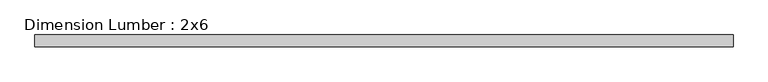
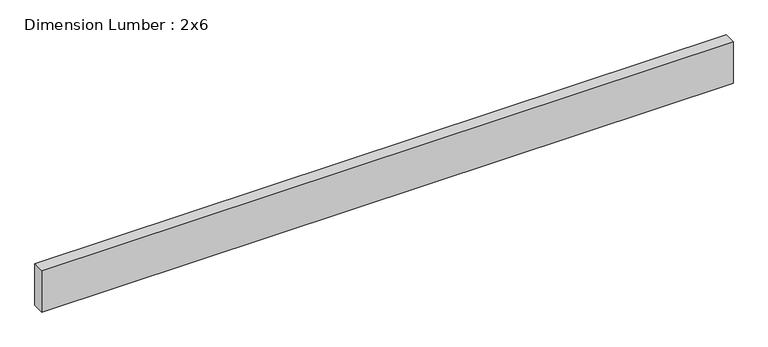
"""IFC4 building model written with IfcOpenShell, lengths in millimetres: beam geometry, Dimension Lumber : 2x6."""

import ifcopenshell
import ifcopenshell.guid

model = None  # the IFC model being written
_history = None  # IfcOwnerHistory: only IFC2X3 demands one
_inside = {}  # id of a spatial element -> (the spatial element, [elements in it])
_under = {}  # id of a project, library or spatial element -> (it, [spatial elements below it])
_declared = {}  # id of a project -> (the project, [libraries it declares])
_typed = {}  # id of a type object -> (the type object, [elements of that type])
_made_of = {}  # id of a material, layer set ... -> (it, [elements and type objects made of it])


def new_model(schema):
    """Start an empty IFC model of exactly this schema.

    Asked for "IFC4X3", IfcOpenShell would pick the latest addendum, in which some entities
    have other attributes; the version numbers below select the first issue.
    IFC2X3 requires an IfcOwnerHistory on every rooted entity: one is made here for all.
    """
    global model, _history
    if schema == "IFC4X3":
        model = ifcopenshell.file(schema_version=(4, 3, 0, 0))
    else:
        model = ifcopenshell.file(schema=schema)
    _inside.clear()
    _under.clear()
    _declared.clear()
    _typed.clear()
    _made_of.clear()
    _history = None
    if model.schema == "IFC2X3":
        org = make("IfcOrganization", Name="unknown")
        user = make(
            "IfcPersonAndOrganization",
            ThePerson=make("IfcPerson", FamilyName="unknown"),
            TheOrganization=org,
        )
        app = make(
            "IfcApplication",
            ApplicationDeveloper=org,
            Version="unknown",
            ApplicationFullName="unknown",
            ApplicationIdentifier="unknown",
        )
        _history = make(
            "IfcOwnerHistory",
            OwningUser=user,
            OwningApplication=app,
            ChangeAction="ADDED",
            CreationDate=0,
        )
    return model


def make(cls, **values):
    """One entity of the class cls with the attributes given. An attribute that is None is left unset."""
    return model.create_entity(
        cls, **{name: value for name, value in values.items() if value is not None}
    )


def rooted(cls, **values):
    """An entity with a GlobalId (a new one), such as an element, a storey or a relation."""
    return make(cls, GlobalId=ifcopenshell.guid.new(), OwnerHistory=_history, **values)


def si_unit(unit_type, name, prefix=None):
    """IfcSIUnit, for example si_unit("LENGTHUNIT", "METRE", prefix="MILLI")."""
    return make("IfcSIUnit", UnitType=unit_type, Prefix=prefix, Name=name)


def assignment(units):
    """IfcUnitAssignment: the units of a project."""
    return None if units is None else make("IfcUnitAssignment", Units=units)


def point(xyz):
    """IfcCartesianPoint."""
    return None if xyz is None else make("IfcCartesianPoint", Coordinates=xyz)


def direction(xyz):
    """IfcDirection."""
    return None if xyz is None else make("IfcDirection", DirectionRatios=xyz)


def frame(location, z_axis=None, x_axis=None):
    """IfcAxis2Placement3D, a coordinate frame: its origin and axes. An axis left out is left unset."""
    return make(
        "IfcAxis2Placement3D",
        Location=point(location),
        Axis=direction(z_axis),
        RefDirection=direction(x_axis),
    )


def origin():
    """The frame at (0, 0, 0) with its axes left unset."""
    return frame((0.0, 0.0, 0.0))


def place(relative_to, where):
    """IfcLocalPlacement: puts the frame where relative to a parent placement (None: the world)."""
    return make(
        "IfcLocalPlacement", PlacementRelTo=relative_to, RelativePlacement=where
    )


def context(
    kind, dimensions, precision=None, world=None, true_north=None, identifier=None
):
    """IfcGeometricRepresentationContext, for example the 3D "Model" context."""
    return make(
        "IfcGeometricRepresentationContext",
        ContextIdentifier=identifier,
        ContextType=kind,
        CoordinateSpaceDimension=dimensions,
        Precision=precision,
        WorldCoordinateSystem=world,
        TrueNorth=true_north,
    )


def project(units=None, contexts=None):
    """IfcProject with its units and contexts."""
    return rooted(
        "IfcProject",
        Name="project",
        RepresentationContexts=contexts,
        UnitsInContext=assignment(units),
    )


def spatial(cls, under=None, at=None, **own):
    """A site, building, storey or space (cls), placed at a placement, below another one or the project."""
    s = rooted(cls, ObjectPlacement=at, **own)
    if under is not None:
        _under.setdefault(under.id(), (under, []))[1].append(s)
    return s


def polyline(points):
    """IfcPolyline through the points."""
    return make("IfcPolyline", Points=[point(p) for p in points])


def outline(outer, holes=None, kind="AREA"):
    """IfcArbitraryClosedProfileDef: a profile drawn as a closed curve; with holes, ...WithVoids."""
    if holes is None:
        return make("IfcArbitraryClosedProfileDef", ProfileType=kind, OuterCurve=outer)
    return make(
        "IfcArbitraryProfileDefWithVoids",
        ProfileType=kind,
        OuterCurve=outer,
        InnerCurves=holes,
    )


def extrude(swept, where, along, depth):
    """IfcExtrudedAreaSolid: the profile swept, set in the frame where, extruded along a direction by depth."""
    return make(
        "IfcExtrudedAreaSolid",
        SweptArea=swept,
        Position=where,
        ExtrudedDirection=direction(along),
        Depth=depth,
    )


def shape(context_of_items, identifier, shape_type, items):
    """IfcShapeRepresentation: the items that make up one representation, for example the "Body"."""
    return make(
        "IfcShapeRepresentation",
        ContextOfItems=context_of_items,
        RepresentationIdentifier=identifier,
        RepresentationType=shape_type,
        Items=items,
    )


def source(mapping_origin, context_of_items, identifier, shape_type, items):
    """IfcRepresentationMap: a shape defined once, which mapped items show again and again."""
    return make(
        "IfcRepresentationMap",
        MappingOrigin=mapping_origin,
        MappedRepresentation=shape(context_of_items, identifier, shape_type, items),
    )


def transform(
    local_origin,
    x_axis=None,
    y_axis=None,
    z_axis=None,
    scale=None,
    scale2=None,
    scale3=None,
    uniform=True,
):
    """IfcCartesianTransformationOperator3D, or its non-uniform kind. x_axis, y_axis, z_axis: its Axis1, 2, 3."""
    if uniform:
        return make(
            "IfcCartesianTransformationOperator3D",
            Axis1=direction(x_axis),
            Axis2=direction(y_axis),
            LocalOrigin=point(local_origin),
            Scale=scale,
            Axis3=direction(z_axis),
        )
    return make(
        "IfcCartesianTransformationOperator3DnonUniform",
        Axis1=direction(x_axis),
        Axis2=direction(y_axis),
        LocalOrigin=point(local_origin),
        Scale=scale,
        Axis3=direction(z_axis),
        Scale2=scale2,
        Scale3=scale3,
    )


def mapped(mapping_source, mapping_target):
    """IfcMappedItem: shows the shape of a source again, moved by a transform."""
    return make(
        "IfcMappedItem", MappingSource=mapping_source, MappingTarget=mapping_target
    )


def made_of(thing, what):
    """Note that an element or type object is made of a material, layer set ...; save() writes the relation."""
    if what is not None:
        _made_of.setdefault(what.id(), (what, []))[1].append(thing)
    return thing


def element(
    cls,
    number,
    at=None,
    inside=None,
    cuts=None,
    type_object=None,
    material=None,
    context=None,
    identifier="Body",
    shape_type=None,
    held_by="IfcProductDefinitionShape",
    body=None,
    shapes=None,
    **own,
):
    """One element of the class cls, such as IfcWall. Its Tag is "e" and its number.

    at: its placement. inside: the storey or other place that contains it. cuts: it is an
    opening in that element (IfcRelVoidsElement). A single representation is given by context,
    identifier, shape_type and body (its items); several are given by shapes. held_by: the class
    of the entity that holds the representations. save() writes the other relations.
    """
    e = rooted(cls, Tag="e%d" % number, ObjectPlacement=at, **own)
    if body is not None:
        shapes = [shape(context, identifier, shape_type, body)]
    if shapes is not None:
        e.Representation = make(held_by, Representations=shapes)
    if inside is not None:
        _inside.setdefault(inside.id(), (inside, []))[1].append(e)
    if cuts is not None:
        rooted(
            "IfcRelVoidsElement", RelatingBuildingElement=cuts, RelatedOpeningElement=e
        )
    if type_object is not None:
        _typed.setdefault(type_object.id(), (type_object, []))[1].append(e)
    return made_of(e, material)


def aggregate(whole, parts):
    """IfcRelAggregates: a whole, such as a stair, and the parts it consists of."""
    return rooted("IfcRelAggregates", RelatingObject=whole, RelatedObjects=parts)


def save(model, path):
    """Write the relations noted so far, then the file.

    IfcRelAggregates (storeys below a building ...), IfcRelContainedInSpatialStructure (elements
    in a storey), IfcRelDefinesByType, IfcRelAssociatesMaterial and IfcRelDeclares: one each for
    every whole, place, type object, material and project.
    """
    for whole, parts in _under.values():
        aggregate(whole, parts)
    for where, things in _inside.values():
        rooted(
            "IfcRelContainedInSpatialStructure",
            RelatedElements=things,
            RelatingStructure=where,
        )
    for kind, things in _typed.values():
        rooted("IfcRelDefinesByType", RelatedObjects=things, RelatingType=kind)
    for what, things in _made_of.values():
        rooted("IfcRelAssociatesMaterial", RelatedObjects=things, RelatingMaterial=what)
    for by, libraries in _declared.values():
        rooted("IfcRelDeclares", RelatingContext=by, RelatedDefinitions=libraries)
    model.write(path)


def dimension_lumber_2x6_f4b49fb7(model_context):
    return source(origin(), model_context, "Body", "SweptSolid", [
        extrude(outline(polyline([(1700.453938, 19.05), (1700.453938, -19.05), (-505.9373564, -19.05), (-505.9373564, 19.05), (1700.453938, 19.05)])), frame((0.0, 0.0, -69.85), z_axis=(0.0, 0.0, 1.0), x_axis=(1.0, 0.0, 0.0)), (0.0, 0.0, 1.0), 139.7),
    ])


if __name__ == "__main__":
    model = new_model("IFC4")
    model_context = context("Model", 3, world=origin())
    ifc_project = project(units=[si_unit("LENGTHUNIT", "METRE", prefix="MILLI")], contexts=[model_context])
    site = spatial("IfcSite", under=ifc_project)
    building = spatial("IfcBuilding", under=site)
    placement = place(None, origin())
    dimension_lumber_2x6_shape = dimension_lumber_2x6_f4b49fb7(model_context)
    element("IfcBeam", 1, ObjectType="Dimension Lumber : 2x6", at=placement, inside=building, context=model_context, shape_type="MappedRepresentation", body=[
        mapped(dimension_lumber_2x6_shape, transform((0.0, 0.0, 0.0), x_axis=(1.0, 0.0, 0.0), y_axis=(0.0, 1.0, 0.0), z_axis=(0.0, 0.0, 1.0))),
    ])
    save(model, "model.ifc")

# Revit data of these elements
# Type "Dimension Lumber : 2x6"
#   Assembly Code = "B10"
#   A = 0.0572917 SF
#   Length [instance default] = 5' - 0"
#   b = 0' - 1 1/2"
#   d = 0' - 5 1/2"
#   Structural Material [instance default] = PRE-ENGINEERED TRUSS @ 24" O.C.
# Element 1 (IfcBeam, "Dimension Lumber : 2x6")
#   Structural Material = 2 X 6 RAFTER BEYOND
#   Materials on its faces: "2 X 6 RAFTER BEYOND"
# Materials
#   "PRE-ENGINEERED TRUSS @ 24\" O.C.": class "Wood", colour RGB 255 255 255, transparency 0, Description = "Pinus Echinata", Cost = 0
#   "2 X 6 RAFTER BEYOND": class "Wood", colour RGB 234 198 147, transparency 0, Description = "Pinus Echinata", Cost = 0
